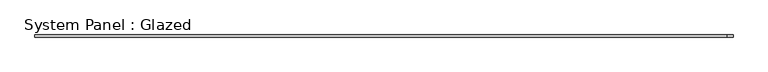
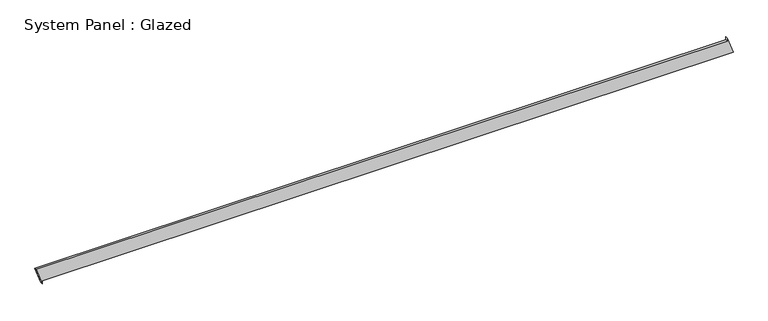
"""IFC4 building model written with IfcOpenShell, lengths in millimetres: plate geometry, System Panel : Glazed."""

import ifcopenshell
import ifcopenshell.guid

model = None  # the IFC model being written
_history = None  # IfcOwnerHistory: only IFC2X3 demands one
_inside = {}  # id of a spatial element -> (the spatial element, [elements in it])
_under = {}  # id of a project, library or spatial element -> (it, [spatial elements below it])
_declared = {}  # id of a project -> (the project, [libraries it declares])
_typed = {}  # id of a type object -> (the type object, [elements of that type])
_made_of = {}  # id of a material, layer set ... -> (it, [elements and type objects made of it])


def new_model(schema):
    """Start an empty IFC model of exactly this schema.

    Asked for "IFC4X3", IfcOpenShell would pick the latest addendum, in which some entities
    have other attributes; the version numbers below select the first issue.
    IFC2X3 requires an IfcOwnerHistory on every rooted entity: one is made here for all.
    """
    global model, _history
    if schema == "IFC4X3":
        model = ifcopenshell.file(schema_version=(4, 3, 0, 0))
    else:
        model = ifcopenshell.file(schema=schema)
    _inside.clear()
    _under.clear()
    _declared.clear()
    _typed.clear()
    _made_of.clear()
    _history = None
    if model.schema == "IFC2X3":
        org = make("IfcOrganization", Name="unknown")
        user = make(
            "IfcPersonAndOrganization",
            ThePerson=make("IfcPerson", FamilyName="unknown"),
            TheOrganization=org,
        )
        app = make(
            "IfcApplication",
            ApplicationDeveloper=org,
            Version="unknown",
            ApplicationFullName="unknown",
            ApplicationIdentifier="unknown",
        )
        _history = make(
            "IfcOwnerHistory",
            OwningUser=user,
            OwningApplication=app,
            ChangeAction="ADDED",
            CreationDate=0,
        )
    return model


def make(cls, **values):
    """One entity of the class cls with the attributes given. An attribute that is None is left unset."""
    return model.create_entity(
        cls, **{name: value for name, value in values.items() if value is not None}
    )


def rooted(cls, **values):
    """An entity with a GlobalId (a new one), such as an element, a storey or a relation."""
    return make(cls, GlobalId=ifcopenshell.guid.new(), OwnerHistory=_history, **values)


def si_unit(unit_type, name, prefix=None):
    """IfcSIUnit, for example si_unit("LENGTHUNIT", "METRE", prefix="MILLI")."""
    return make("IfcSIUnit", UnitType=unit_type, Prefix=prefix, Name=name)


def assignment(units):
    """IfcUnitAssignment: the units of a project."""
    return None if units is None else make("IfcUnitAssignment", Units=units)


def point(xyz):
    """IfcCartesianPoint."""
    return None if xyz is None else make("IfcCartesianPoint", Coordinates=xyz)


def direction(xyz):
    """IfcDirection."""
    return None if xyz is None else make("IfcDirection", DirectionRatios=xyz)


def frame(location, z_axis=None, x_axis=None):
    """IfcAxis2Placement3D, a coordinate frame: its origin and axes. An axis left out is left unset."""
    return make(
        "IfcAxis2Placement3D",
        Location=point(location),
        Axis=direction(z_axis),
        RefDirection=direction(x_axis),
    )


def origin():
    """The frame at (0, 0, 0) with its axes left unset."""
    return frame((0.0, 0.0, 0.0))


def place(relative_to, where):
    """IfcLocalPlacement: puts the frame where relative to a parent placement (None: the world)."""
    return make(
        "IfcLocalPlacement", PlacementRelTo=relative_to, RelativePlacement=where
    )


def context(
    kind, dimensions, precision=None, world=None, true_north=None, identifier=None
):
    """IfcGeometricRepresentationContext, for example the 3D "Model" context."""
    return make(
        "IfcGeometricRepresentationContext",
        ContextIdentifier=identifier,
        ContextType=kind,
        CoordinateSpaceDimension=dimensions,
        Precision=precision,
        WorldCoordinateSystem=world,
        TrueNorth=true_north,
    )


def project(units=None, contexts=None):
    """IfcProject with its units and contexts."""
    return rooted(
        "IfcProject",
        Name="project",
        RepresentationContexts=contexts,
        UnitsInContext=assignment(units),
    )


def spatial(cls, under=None, at=None, **own):
    """A site, building, storey or space (cls), placed at a placement, below another one or the project."""
    s = rooted(cls, ObjectPlacement=at, **own)
    if under is not None:
        _under.setdefault(under.id(), (under, []))[1].append(s)
    return s


def polyline(points):
    """IfcPolyline through the points."""
    return make("IfcPolyline", Points=[point(p) for p in points])


def outline(outer, holes=None, kind="AREA"):
    """IfcArbitraryClosedProfileDef: a profile drawn as a closed curve; with holes, ...WithVoids."""
    if holes is None:
        return make("IfcArbitraryClosedProfileDef", ProfileType=kind, OuterCurve=outer)
    return make(
        "IfcArbitraryProfileDefWithVoids",
        ProfileType=kind,
        OuterCurve=outer,
        InnerCurves=holes,
    )


def extrude(swept, where, along, depth):
    """IfcExtrudedAreaSolid: the profile swept, set in the frame where, extruded along a direction by depth."""
    return make(
        "IfcExtrudedAreaSolid",
        SweptArea=swept,
        Position=where,
        ExtrudedDirection=direction(along),
        Depth=depth,
    )


def shape(context_of_items, identifier, shape_type, items):
    """IfcShapeRepresentation: the items that make up one representation, for example the "Body"."""
    return make(
        "IfcShapeRepresentation",
        ContextOfItems=context_of_items,
        RepresentationIdentifier=identifier,
        RepresentationType=shape_type,
        Items=items,
    )


def source(mapping_origin, context_of_items, identifier, shape_type, items):
    """IfcRepresentationMap: a shape defined once, which mapped items show again and again."""
    return make(
        "IfcRepresentationMap",
        MappingOrigin=mapping_origin,
        MappedRepresentation=shape(context_of_items, identifier, shape_type, items),
    )


def transform(
    local_origin,
    x_axis=None,
    y_axis=None,
    z_axis=None,
    scale=None,
    scale2=None,
    scale3=None,
    uniform=True,
):
    """IfcCartesianTransformationOperator3D, or its non-uniform kind. x_axis, y_axis, z_axis: its Axis1, 2, 3."""
    if uniform:
        return make(
            "IfcCartesianTransformationOperator3D",
            Axis1=direction(x_axis),
            Axis2=direction(y_axis),
            LocalOrigin=point(local_origin),
            Scale=scale,
            Axis3=direction(z_axis),
        )
    return make(
        "IfcCartesianTransformationOperator3DnonUniform",
        Axis1=direction(x_axis),
        Axis2=direction(y_axis),
        LocalOrigin=point(local_origin),
        Scale=scale,
        Axis3=direction(z_axis),
        Scale2=scale2,
        Scale3=scale3,
    )


def mapped(mapping_source, mapping_target):
    """IfcMappedItem: shows the shape of a source again, moved by a transform."""
    return make(
        "IfcMappedItem", MappingSource=mapping_source, MappingTarget=mapping_target
    )


def made_of(thing, what):
    """Note that an element or type object is made of a material, layer set ...; save() writes the relation."""
    if what is not None:
        _made_of.setdefault(what.id(), (what, []))[1].append(thing)
    return thing


def element(
    cls,
    number,
    at=None,
    inside=None,
    cuts=None,
    type_object=None,
    material=None,
    context=None,
    identifier="Body",
    shape_type=None,
    held_by="IfcProductDefinitionShape",
    body=None,
    shapes=None,
    **own,
):
    """One element of the class cls, such as IfcWall. Its Tag is "e" and its number.

    at: its placement. inside: the storey or other place that contains it. cuts: it is an
    opening in that element (IfcRelVoidsElement). A single representation is given by context,
    identifier, shape_type and body (its items); several are given by shapes. held_by: the class
    of the entity that holds the representations. save() writes the other relations.
    """
    e = rooted(cls, Tag="e%d" % number, ObjectPlacement=at, **own)
    if body is not None:
        shapes = [shape(context, identifier, shape_type, body)]
    if shapes is not None:
        e.Representation = make(held_by, Representations=shapes)
    if inside is not None:
        _inside.setdefault(inside.id(), (inside, []))[1].append(e)
    if cuts is not None:
        rooted(
            "IfcRelVoidsElement", RelatingBuildingElement=cuts, RelatedOpeningElement=e
        )
    if type_object is not None:
        _typed.setdefault(type_object.id(), (type_object, []))[1].append(e)
    return made_of(e, material)


def aggregate(whole, parts):
    """IfcRelAggregates: a whole, such as a stair, and the parts it consists of."""
    return rooted("IfcRelAggregates", RelatingObject=whole, RelatedObjects=parts)


def save(model, path):
    """Write the relations noted so far, then the file.

    IfcRelAggregates (storeys below a building ...), IfcRelContainedInSpatialStructure (elements
    in a storey), IfcRelDefinesByType, IfcRelAssociatesMaterial and IfcRelDeclares: one each for
    every whole, place, type object, material and project.
    """
    for whole, parts in _under.values():
        aggregate(whole, parts)
    for where, things in _inside.values():
        rooted(
            "IfcRelContainedInSpatialStructure",
            RelatedElements=things,
            RelatingStructure=where,
        )
    for kind, things in _typed.values():
        rooted("IfcRelDefinesByType", RelatedObjects=things, RelatingType=kind)
    for what, things in _made_of.values():
        rooted("IfcRelAssociatesMaterial", RelatedObjects=things, RelatingMaterial=what)
    for by, libraries in _declared.values():
        rooted("IfcRelDeclares", RelatingContext=by, RelatedDefinitions=libraries)
    model.write(path)


def system_panel_glazed_7537b497(model_context):
    return source(origin(), model_context, "Body", "SweptSolid", [
        extrude(outline(polyline([(0.0, -3959.0229169), (35.3553391, -3959.0229169), (35.3553391, 4028.0764592), (234.64232, 3959.1368322), (199.2869809, 3959.1370419), (199.2396119, -4028.0764592), (0.0, -3959.0229169)])), frame((0.0, -49.5, 0.0), z_axis=(0.0, 1.0, 0.0), x_axis=(0.0, 0.0, 1.0)), (0.0, 0.0, 1.0), 25.0),
    ])


if __name__ == "__main__":
    model = new_model("IFC4")
    model_context = context("Model", 3, world=origin())
    ifc_project = project(units=[si_unit("LENGTHUNIT", "METRE", prefix="MILLI")], contexts=[model_context])
    site = spatial("IfcSite", under=ifc_project)
    building = spatial("IfcBuilding", under=site)
    placement = place(None, origin())
    system_panel_glazed_shape = system_panel_glazed_7537b497(model_context)
    element("IfcPlate", 1, ObjectType="System Panel : Glazed", at=placement, inside=building, context=model_context, shape_type="MappedRepresentation", body=[
        mapped(system_panel_glazed_shape, transform((0.0, 0.0, 0.0), x_axis=(1.0, 0.0, 0.0), y_axis=(0.0, 1.0, 0.0), z_axis=(0.0, 0.0, 1.0))),
    ])
    save(model, "model.ifc")

# Revit data of these elements
# Element 1 (IfcPlate, "System Panel : Glazed")
#   Materials on its faces: "Glass"
# Materials
#   "Glass": class "Glass", colour RGB 218 227 224, transparency 0.85, Description = "Soda Lime Glass", Cost = 0
